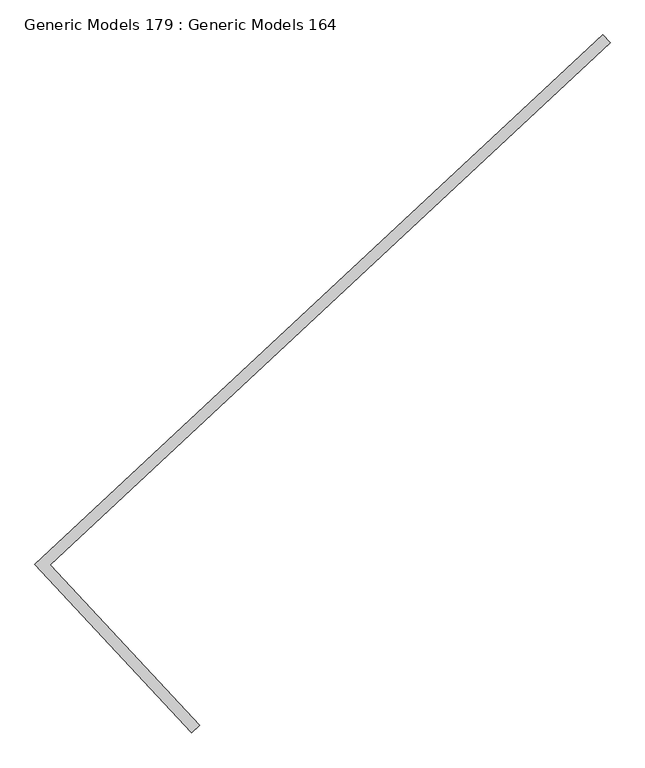
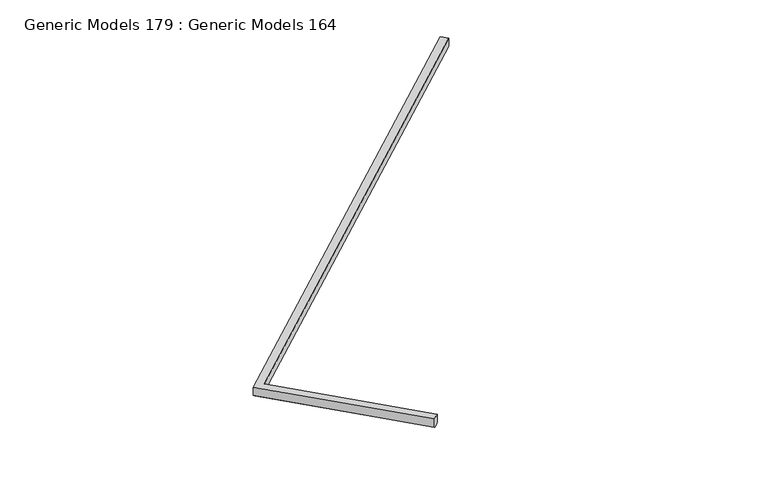
"""IFC4 building model written with IfcOpenShell, lengths in millimetres: proxy geometry, Generic Models 179 : Generic Models 164."""

from ifc_helpers import new_model, si_unit, origin, place, context, project, spatial, faceted_brep, source, transform, mapped, element, save


def generic_models_179_generic_models_164_c2fe7096(model_context):
    return source(origin(), model_context, "Body", "Brep", [
        faceted_brep([(3995.8871222, -24546.512996, 2239.565625), (3903.0052021, -24633.1267877, 2239.565625), (3903.0052021, -24633.1267877, 2099.865625), (3916.9374901, -24620.134719, 2099.865625), (3916.9374901, -24620.134719, 2082.8), (3981.9548342, -24559.5050647, 2082.8), (3981.9548342, -24559.5050647, 2099.865625), (3995.8871222, -24546.512996, 2099.865625), (2089.3864847, -22660.3262047, 2082.8), (8739.7319642, -16458.778717, 2082.8), (8800.3616184, -16523.7960611, 2082.8), (2215.033483, -22664.7138946, 2082.8), (2062.4621279, -22659.3859855, 2099.865625), (8726.7398955, -16444.846429, 2099.865625), (8739.7319642, -16458.778717, 2099.865625), (2089.3864847, -22660.3262047, 2099.865625), (2215.033483, -22664.7138946, 2099.865625), (8800.3616184, -16523.7960611, 2099.865625), (8813.3536872, -16537.7283491, 2099.865625), (2241.9578397, -22665.6541138, 2099.865625), (2062.4621279, -22659.3859855, 2239.565625), (8813.3536872, -16537.7283491, 2239.565625), (8726.7398955, -16444.846429, 2239.565625), (2241.9578397, -22665.6541138, 2239.565625)], [[[0, 1, 2, 3, 4, 5, 6, 7]], [[5, 4, 8, 9, 10, 11]], [[3, 2, 12, 13, 14, 15]], [[4, 3, 15, 8]], [[7, 6, 16, 17, 18, 19]], [[6, 5, 11, 16]], [[2, 1, 20, 12]], [[21, 18, 17, 10, 9, 14, 13, 22]], [[8, 15, 14, 9]], [[16, 11, 10, 17]], [[12, 20, 22, 13]], [[1, 0, 23, 21, 22, 20]], [[0, 7, 19, 23]], [[23, 19, 18, 21]]]),
    ])


if __name__ == "__main__":
    model = new_model("IFC4")
    model_context = context("Model", 3, world=origin())
    ifc_project = project(units=[si_unit("LENGTHUNIT", "METRE", prefix="MILLI")], contexts=[model_context])
    site = spatial("IfcSite", under=ifc_project)
    building = spatial("IfcBuilding", under=site)
    placement = place(None, origin())
    generic_models_179_generic_models_164_shape = generic_models_179_generic_models_164_c2fe7096(model_context)
    element("IfcBuildingElementProxy", 1, Name="Generic Models 179 : Generic Models 164", ObjectType="Generic Models 179 : Generic Models 164", at=placement, inside=building, context=model_context, shape_type="MappedRepresentation", body=[
        mapped(generic_models_179_generic_models_164_shape, transform((0.0, 0.0, 0.0), x_axis=(1.0, 0.0, 0.0), y_axis=(0.0, 1.0, 0.0), z_axis=(0.0, 0.0, 1.0))),
    ])
    save(model, "model.ifc")

# Revit data of these elements
# Element 1 (IfcBuildingElementProxy, "Generic Models 179 : Generic Models 164")
#   Materials on its faces: "1 x 6 WOOD TRIM"
# Materials
#   "1 x 6 WOOD TRIM": class "Wood", colour RGB 48 37 22, transparency 0, Description = "Pinus Echinata", Cost = 0
